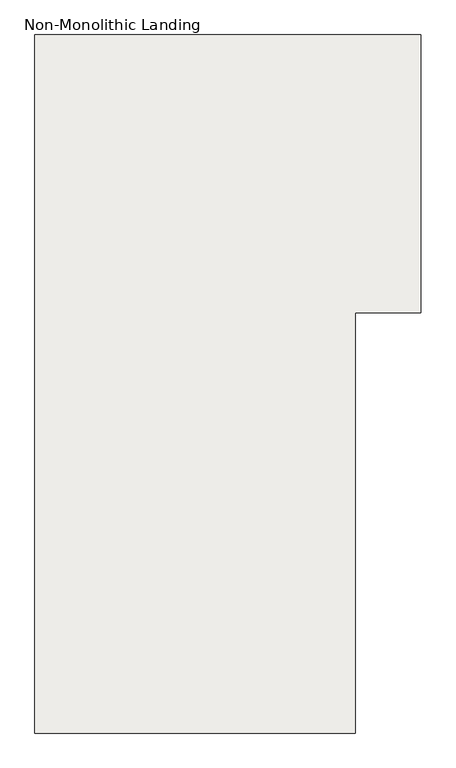
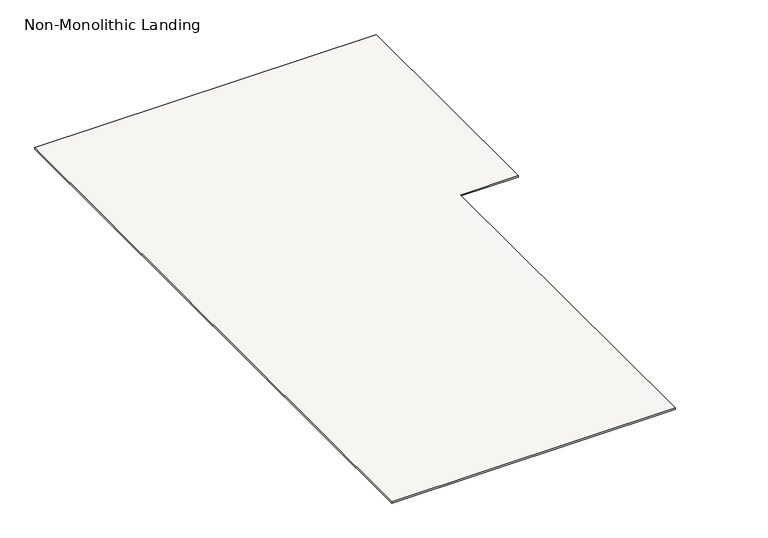
"""IFC4 building model written with IfcOpenShell, lengths in millimetres: slab geometry, Non-Monolithic Landing."""

import ifcopenshell
import ifcopenshell.guid

model = None  # the IFC model being written
_history = None  # IfcOwnerHistory: only IFC2X3 demands one
_inside = {}  # id of a spatial element -> (the spatial element, [elements in it])
_under = {}  # id of a project, library or spatial element -> (it, [spatial elements below it])
_declared = {}  # id of a project -> (the project, [libraries it declares])
_typed = {}  # id of a type object -> (the type object, [elements of that type])
_made_of = {}  # id of a material, layer set ... -> (it, [elements and type objects made of it])


def new_model(schema):
    """Start an empty IFC model of exactly this schema.

    Asked for "IFC4X3", IfcOpenShell would pick the latest addendum, in which some entities
    have other attributes; the version numbers below select the first issue.
    IFC2X3 requires an IfcOwnerHistory on every rooted entity: one is made here for all.
    """
    global model, _history
    if schema == "IFC4X3":
        model = ifcopenshell.file(schema_version=(4, 3, 0, 0))
    else:
        model = ifcopenshell.file(schema=schema)
    _inside.clear()
    _under.clear()
    _declared.clear()
    _typed.clear()
    _made_of.clear()
    _history = None
    if model.schema == "IFC2X3":
        org = make("IfcOrganization", Name="unknown")
        user = make(
            "IfcPersonAndOrganization",
            ThePerson=make("IfcPerson", FamilyName="unknown"),
            TheOrganization=org,
        )
        app = make(
            "IfcApplication",
            ApplicationDeveloper=org,
            Version="unknown",
            ApplicationFullName="unknown",
            ApplicationIdentifier="unknown",
        )
        _history = make(
            "IfcOwnerHistory",
            OwningUser=user,
            OwningApplication=app,
            ChangeAction="ADDED",
            CreationDate=0,
        )
    return model


def make(cls, **values):
    """One entity of the class cls with the attributes given. An attribute that is None is left unset."""
    return model.create_entity(
        cls, **{name: value for name, value in values.items() if value is not None}
    )


def rooted(cls, **values):
    """An entity with a GlobalId (a new one), such as an element, a storey or a relation."""
    return make(cls, GlobalId=ifcopenshell.guid.new(), OwnerHistory=_history, **values)


def si_unit(unit_type, name, prefix=None):
    """IfcSIUnit, for example si_unit("LENGTHUNIT", "METRE", prefix="MILLI")."""
    return make("IfcSIUnit", UnitType=unit_type, Prefix=prefix, Name=name)


def assignment(units):
    """IfcUnitAssignment: the units of a project."""
    return None if units is None else make("IfcUnitAssignment", Units=units)


def point(xyz):
    """IfcCartesianPoint."""
    return None if xyz is None else make("IfcCartesianPoint", Coordinates=xyz)


def direction(xyz):
    """IfcDirection."""
    return None if xyz is None else make("IfcDirection", DirectionRatios=xyz)


def frame(location, z_axis=None, x_axis=None):
    """IfcAxis2Placement3D, a coordinate frame: its origin and axes. An axis left out is left unset."""
    return make(
        "IfcAxis2Placement3D",
        Location=point(location),
        Axis=direction(z_axis),
        RefDirection=direction(x_axis),
    )


def origin():
    """The frame at (0, 0, 0) with its axes left unset."""
    return frame((0.0, 0.0, 0.0))


def place(relative_to, where):
    """IfcLocalPlacement: puts the frame where relative to a parent placement (None: the world)."""
    return make(
        "IfcLocalPlacement", PlacementRelTo=relative_to, RelativePlacement=where
    )


def context(
    kind, dimensions, precision=None, world=None, true_north=None, identifier=None
):
    """IfcGeometricRepresentationContext, for example the 3D "Model" context."""
    return make(
        "IfcGeometricRepresentationContext",
        ContextIdentifier=identifier,
        ContextType=kind,
        CoordinateSpaceDimension=dimensions,
        Precision=precision,
        WorldCoordinateSystem=world,
        TrueNorth=true_north,
    )


def project(units=None, contexts=None):
    """IfcProject with its units and contexts."""
    return rooted(
        "IfcProject",
        Name="project",
        RepresentationContexts=contexts,
        UnitsInContext=assignment(units),
    )


def spatial(cls, under=None, at=None, **own):
    """A site, building, storey or space (cls), placed at a placement, below another one or the project."""
    s = rooted(cls, ObjectPlacement=at, **own)
    if under is not None:
        _under.setdefault(under.id(), (under, []))[1].append(s)
    return s


def polyline(points):
    """IfcPolyline through the points."""
    return make("IfcPolyline", Points=[point(p) for p in points])


def outline(outer, holes=None, kind="AREA"):
    """IfcArbitraryClosedProfileDef: a profile drawn as a closed curve; with holes, ...WithVoids."""
    if holes is None:
        return make("IfcArbitraryClosedProfileDef", ProfileType=kind, OuterCurve=outer)
    return make(
        "IfcArbitraryProfileDefWithVoids",
        ProfileType=kind,
        OuterCurve=outer,
        InnerCurves=holes,
    )


def extrude(swept, where, along, depth):
    """IfcExtrudedAreaSolid: the profile swept, set in the frame where, extruded along a direction by depth."""
    return make(
        "IfcExtrudedAreaSolid",
        SweptArea=swept,
        Position=where,
        ExtrudedDirection=direction(along),
        Depth=depth,
    )


def shape(context_of_items, identifier, shape_type, items):
    """IfcShapeRepresentation: the items that make up one representation, for example the "Body"."""
    return make(
        "IfcShapeRepresentation",
        ContextOfItems=context_of_items,
        RepresentationIdentifier=identifier,
        RepresentationType=shape_type,
        Items=items,
    )


def source(mapping_origin, context_of_items, identifier, shape_type, items):
    """IfcRepresentationMap: a shape defined once, which mapped items show again and again."""
    return make(
        "IfcRepresentationMap",
        MappingOrigin=mapping_origin,
        MappedRepresentation=shape(context_of_items, identifier, shape_type, items),
    )


def transform(
    local_origin,
    x_axis=None,
    y_axis=None,
    z_axis=None,
    scale=None,
    scale2=None,
    scale3=None,
    uniform=True,
):
    """IfcCartesianTransformationOperator3D, or its non-uniform kind. x_axis, y_axis, z_axis: its Axis1, 2, 3."""
    if uniform:
        return make(
            "IfcCartesianTransformationOperator3D",
            Axis1=direction(x_axis),
            Axis2=direction(y_axis),
            LocalOrigin=point(local_origin),
            Scale=scale,
            Axis3=direction(z_axis),
        )
    return make(
        "IfcCartesianTransformationOperator3DnonUniform",
        Axis1=direction(x_axis),
        Axis2=direction(y_axis),
        LocalOrigin=point(local_origin),
        Scale=scale,
        Axis3=direction(z_axis),
        Scale2=scale2,
        Scale3=scale3,
    )


def mapped(mapping_source, mapping_target):
    """IfcMappedItem: shows the shape of a source again, moved by a transform."""
    return make(
        "IfcMappedItem", MappingSource=mapping_source, MappingTarget=mapping_target
    )


def made_of(thing, what):
    """Note that an element or type object is made of a material, layer set ...; save() writes the relation."""
    if what is not None:
        _made_of.setdefault(what.id(), (what, []))[1].append(thing)
    return thing


def element(
    cls,
    number,
    at=None,
    inside=None,
    cuts=None,
    type_object=None,
    material=None,
    context=None,
    identifier="Body",
    shape_type=None,
    held_by="IfcProductDefinitionShape",
    body=None,
    shapes=None,
    **own,
):
    """One element of the class cls, such as IfcWall. Its Tag is "e" and its number.

    at: its placement. inside: the storey or other place that contains it. cuts: it is an
    opening in that element (IfcRelVoidsElement). A single representation is given by context,
    identifier, shape_type and body (its items); several are given by shapes. held_by: the class
    of the entity that holds the representations. save() writes the other relations.
    """
    e = rooted(cls, Tag="e%d" % number, ObjectPlacement=at, **own)
    if body is not None:
        shapes = [shape(context, identifier, shape_type, body)]
    if shapes is not None:
        e.Representation = make(held_by, Representations=shapes)
    if inside is not None:
        _inside.setdefault(inside.id(), (inside, []))[1].append(e)
    if cuts is not None:
        rooted(
            "IfcRelVoidsElement", RelatingBuildingElement=cuts, RelatedOpeningElement=e
        )
    if type_object is not None:
        _typed.setdefault(type_object.id(), (type_object, []))[1].append(e)
    return made_of(e, material)


def aggregate(whole, parts):
    """IfcRelAggregates: a whole, such as a stair, and the parts it consists of."""
    return rooted("IfcRelAggregates", RelatingObject=whole, RelatedObjects=parts)


def save(model, path):
    """Write the relations noted so far, then the file.

    IfcRelAggregates (storeys below a building ...), IfcRelContainedInSpatialStructure (elements
    in a storey), IfcRelDefinesByType, IfcRelAssociatesMaterial and IfcRelDeclares: one each for
    every whole, place, type object, material and project.
    """
    for whole, parts in _under.values():
        aggregate(whole, parts)
    for where, things in _inside.values():
        rooted(
            "IfcRelContainedInSpatialStructure",
            RelatedElements=things,
            RelatingStructure=where,
        )
    for kind, things in _typed.values():
        rooted("IfcRelDefinesByType", RelatedObjects=things, RelatingType=kind)
    for what, things in _made_of.values():
        rooted("IfcRelAssociatesMaterial", RelatedObjects=things, RelatingMaterial=what)
    for by, libraries in _declared.values():
        rooted("IfcRelDeclares", RelatingContext=by, RelatedDefinitions=libraries)
    model.write(path)


def non_monolithic_landing_f936f41c(model_context):
    return source(origin(), model_context, "Body", "SweptSolid", [
        extrude(outline(polyline([(12231.0, 13220.4345331), (13883.4671154, 13220.4345331), (13883.4671154, 12030.4345331), (13603.0, 12030.4345331), (13603.0, 10230.4345331), (12231.0, 10230.4345331), (12231.0, 13220.4345331)])), frame((0.0, 0.0, 7994.0), z_axis=(0.0, 0.0, 1.0), x_axis=(1.0, 0.0, 0.0)), (0.0, 0.0, 1.0), 6.0),
    ])


if __name__ == "__main__":
    model = new_model("IFC4")
    model_context = context("Model", 3, world=origin())
    ifc_project = project(units=[si_unit("LENGTHUNIT", "METRE", prefix="MILLI")], contexts=[model_context])
    site = spatial("IfcSite", under=ifc_project)
    building = spatial("IfcBuilding", under=site)
    placement = place(None, origin())
    non_monolithic_landing_shape = non_monolithic_landing_f936f41c(model_context)
    element("IfcSlab", 1, ObjectType="Non-Monolithic Landing", at=placement, inside=building, context=model_context, shape_type="MappedRepresentation", body=[
        mapped(non_monolithic_landing_shape, transform((0.0, 0.0, 0.0), x_axis=(1.0, 0.0, 0.0), y_axis=(0.0, 1.0, 0.0), z_axis=(0.0, 0.0, 1.0))),
    ])
    save(model, "model.ifc")

# Revit data of these elements
# Element 1 (IfcSlab, "Non-Monolithic Landing")
#   Materials on its faces: "Steel, Paint Finish, Dark Gray"
# Materials
#   "Steel, Paint Finish, Dark Gray": class "Metal", colour RGB 89 89 89, transparency 0, Description = "Steel, paint finish, dark gray, glossy", Cost = 0
